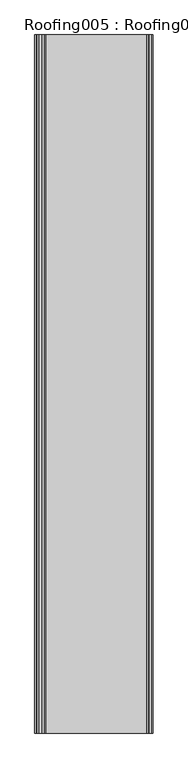
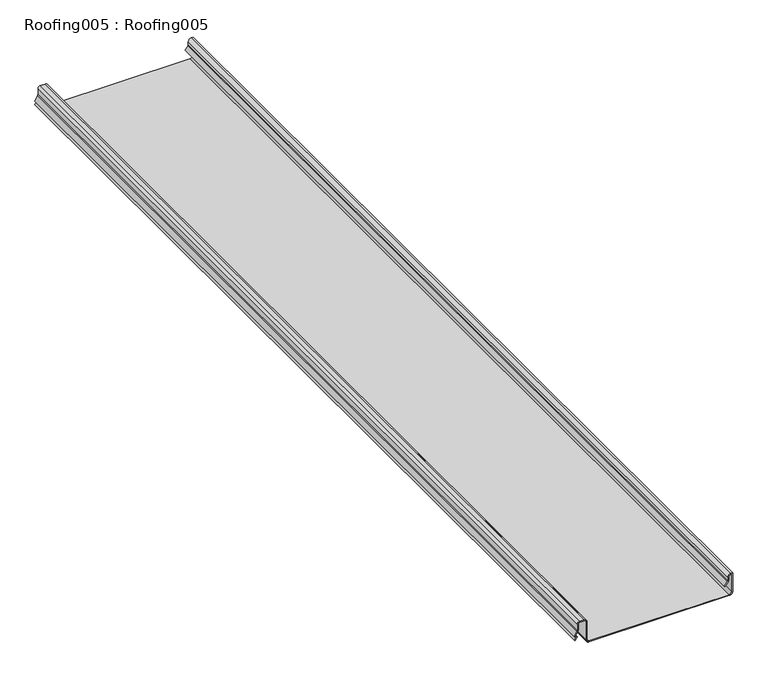
"""IFC4 building model written with IfcOpenShell, lengths in millimetres: proxy geometry, Roofing005 : Roofing005."""

from ifc_helpers import new_model, si_unit, point, frame, frame_2d, origin, place, context, project, spatial, polyline, circle_curve, trimmed, segment, composite_curve, outline, extrude, source, transform, mapped, element, save


def roofing005_roofing005_59f0b18c(model_context):
    return source(origin(), model_context, "Body", "SweptSolid", [
        extrude(outline(composite_curve([segment(trimmed(circle_curve(frame_2d((42571.8416239, -1490.700033)), 5.08), [point((42568.8585944, -1486.588107))], [point((42571.8416239, -1485.620033))], False, "CARTESIAN"), True, "CONTINUOUS"), segment(polyline([(42571.8416239, -1485.620033), (42578.5981823, -1485.620033)]), True, "CONTINUOUS"), segment(trimmed(circle_curve(frame_2d((42578.5981823, -1480.540033)), 5.08), [point((42578.5981823, -1485.620033))], [point((42583.6781823, -1480.540033))], True, "CARTESIAN"), True, "CONTINUOUS"), segment(polyline([(42583.6781823, -1480.540033), (42583.6781823, -1478.9452283), (42543.9409948, -1478.9452283)]), True, "CONTINUOUS"), segment(trimmed(circle_curve(frame_2d((42543.9409948, -1484.0252283)), 5.08), [point((42543.9409948, -1478.9452283))], [point((42538.8609948, -1484.0252283))], True, "CARTESIAN"), True, "CONTINUOUS"), segment(polyline([(42538.8609948, -1484.0252283), (42538.8609948, -1784.2993103)]), True, "CONTINUOUS"), segment(trimmed(circle_curve(frame_2d((42543.9409948, -1784.2993103)), 5.08), [point((42538.8609948, -1784.2993103))], [point((42543.9409948, -1789.3793103))], True, "CARTESIAN"), True, "CONTINUOUS"), segment(polyline([(42543.9409948, -1789.3793103), (42585.5544323, -1789.3793103)]), True, "CONTINUOUS"), segment(trimmed(circle_curve(frame_2d((42585.5544323, -1794.4593103)), 5.08), [point((42585.5544323, -1789.3793103))], [point((42590.6344323, -1794.4593103))], False, "CARTESIAN"), True, "CONTINUOUS"), segment(polyline([(42590.6344323, -1794.4593103), (42590.6344323, -1804.4670872)]), True, "CONTINUOUS"), segment(trimmed(circle_curve(frame_2d((42585.5544323, -1804.4670872)), 5.08), [point((42590.6344323, -1804.4670872))], [point((42585.5544323, -1809.5470872))], False, "CARTESIAN"), True, "CONTINUOUS"), segment(polyline([(42585.5544323, -1809.5470872), (42572.3718581, -1809.5470872)]), True, "CONTINUOUS"), segment(trimmed(circle_curve(frame_2d((42572.3718581, -1814.6270872)), 5.08), [point((42572.3718581, -1809.5470872))], [point((42569.8678467, -1810.2070955))], True, "CARTESIAN"), True, "CONTINUOUS"), segment(polyline([(42569.8678467, -1810.2070955), (42559.3102135, -1816.1882005), (42556.8688073, -1812.024138), (42551.2672448, -1816.0231614), (42550.1051711, -1814.3954069), (42557.4874863, -1809.1250826), (42560.0388845, -1813.4767474), (42568.8820154, -1808.4669413)]), True, "CONTINUOUS"), segment(trimmed(circle_curve(frame_2d((42572.3718581, -1814.6270872)), 7.08), [point((42568.8820154, -1808.4669413))], [point((42572.3718581, -1807.5470872))], False, "CARTESIAN"), True, "CONTINUOUS"), segment(polyline([(42572.3718581, -1807.5470872), (42585.5544323, -1807.5470872)]), True, "CONTINUOUS"), segment(trimmed(circle_curve(frame_2d((42585.5544323, -1804.4670872)), 3.08), [point((42585.5544323, -1807.5470872))], [point((42588.6344323, -1804.4670872))], True, "CARTESIAN"), True, "CONTINUOUS"), segment(polyline([(42588.6344323, -1804.4670872), (42588.6344323, -1794.4593103)]), True, "CONTINUOUS"), segment(trimmed(circle_curve(frame_2d((42585.5544323, -1794.4593103)), 3.08), [point((42588.6344323, -1794.4593103))], [point((42585.5544323, -1791.3793103))], True, "CARTESIAN"), True, "CONTINUOUS"), segment(polyline([(42585.5544323, -1791.3793103), (42543.9409948, -1791.3793103)]), True, "CONTINUOUS"), segment(trimmed(circle_curve(frame_2d((42543.9409948, -1784.2993103)), 7.08), [point((42543.9409948, -1791.3793103))], [point((42536.8609948, -1784.2993103))], False, "CARTESIAN"), True, "CONTINUOUS"), segment(polyline([(42536.8609948, -1784.2993103), (42536.8609948, -1484.0252283)]), True, "CONTINUOUS"), segment(trimmed(circle_curve(frame_2d((42543.9409948, -1484.0252283)), 7.08), [point((42536.8609948, -1484.0252283))], [point((42543.9409948, -1476.9452283))], False, "CARTESIAN"), True, "CONTINUOUS"), segment(polyline([(42543.9409948, -1476.9452283), (42585.6781823, -1476.9452283), (42585.6781823, -1480.540033)]), True, "CONTINUOUS"), segment(trimmed(circle_curve(frame_2d((42578.5981823, -1480.540033)), 7.08), [point((42585.6781823, -1480.540033))], [point((42578.5981823, -1487.620033))], False, "CARTESIAN"), True, "CONTINUOUS"), segment(polyline([(42578.5981823, -1487.620033), (42571.8416239, -1487.620033)]), True, "CONTINUOUS"), segment(trimmed(circle_curve(frame_2d((42571.8416239, -1490.700033)), 3.08), [point((42571.8416239, -1487.620033))], [point((42570.0330155, -1488.2069755))], True, "CARTESIAN"), True, "CONTINUOUS"), segment(polyline([(42570.0330155, -1488.2069755), (42561.5588533, -1494.3546241), (42560.3844323, -1492.7357556), (42568.8585944, -1486.588107)]), True, "CONTINUOUS")], self_intersect=False)), frame((0.0, -1052.8906574, 0.0), z_axis=(0.0, 1.0, 0.0), x_axis=(0.0, 0.0, 1.0)), (0.0, 0.0, 1.0), 2000.0),
    ])


if __name__ == "__main__":
    model = new_model("IFC4")
    model_context = context("Model", 3, world=origin())
    ifc_project = project(units=[si_unit("LENGTHUNIT", "METRE", prefix="MILLI")], contexts=[model_context])
    site = spatial("IfcSite", under=ifc_project)
    building = spatial("IfcBuilding", under=site)
    placement = place(None, origin())
    roofing005_roofing005_shape = roofing005_roofing005_59f0b18c(model_context)
    element("IfcBuildingElementProxy", 1, Name="Roofing005 : Roofing005", ObjectType="Roofing005 : Roofing005", at=placement, inside=building, context=model_context, shape_type="MappedRepresentation", body=[
        mapped(roofing005_roofing005_shape, transform((0.0, 0.0, 0.0), x_axis=(1.0, 0.0, 0.0), y_axis=(0.0, 1.0, 0.0), z_axis=(0.0, 0.0, 1.0))),
    ])
    save(model, "model.ifc")

# Revit data of these elements
# Type "Roofing005 : Roofing005"
#   NameOverride = "Roofing005"
# Element 1 (IfcBuildingElementProxy, "Roofing005 : Roofing005")
#   Materials on its faces: "STANDING SEAM METAL ROOF"
# Materials
#   "STANDING SEAM METAL ROOF": class "Unassigned", colour RGB 128 128 128, transparency 0
